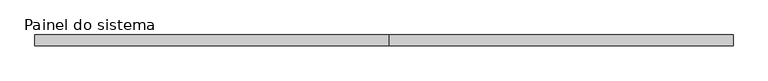
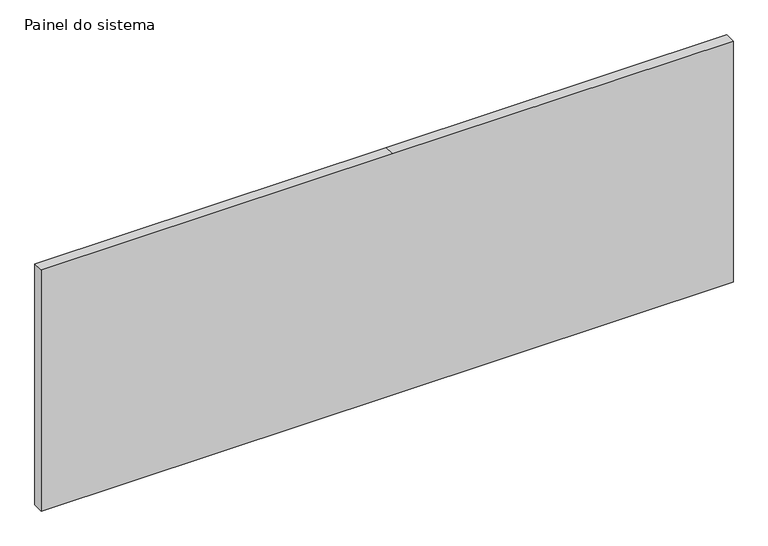
"""IFC4 building model written with IfcOpenShell, lengths in millimetres: plate geometry, Painel do sistema : Envidraçado."""

import ifcopenshell
import ifcopenshell.guid

model = None  # the IFC model being written
_history = None  # IfcOwnerHistory: only IFC2X3 demands one
_inside = {}  # id of a spatial element -> (the spatial element, [elements in it])
_under = {}  # id of a project, library or spatial element -> (it, [spatial elements below it])
_declared = {}  # id of a project -> (the project, [libraries it declares])
_typed = {}  # id of a type object -> (the type object, [elements of that type])
_made_of = {}  # id of a material, layer set ... -> (it, [elements and type objects made of it])


def new_model(schema):
    """Start an empty IFC model of exactly this schema.

    Asked for "IFC4X3", IfcOpenShell would pick the latest addendum, in which some entities
    have other attributes; the version numbers below select the first issue.
    IFC2X3 requires an IfcOwnerHistory on every rooted entity: one is made here for all.
    """
    global model, _history
    if schema == "IFC4X3":
        model = ifcopenshell.file(schema_version=(4, 3, 0, 0))
    else:
        model = ifcopenshell.file(schema=schema)
    _inside.clear()
    _under.clear()
    _declared.clear()
    _typed.clear()
    _made_of.clear()
    _history = None
    if model.schema == "IFC2X3":
        org = make("IfcOrganization", Name="unknown")
        user = make(
            "IfcPersonAndOrganization",
            ThePerson=make("IfcPerson", FamilyName="unknown"),
            TheOrganization=org,
        )
        app = make(
            "IfcApplication",
            ApplicationDeveloper=org,
            Version="unknown",
            ApplicationFullName="unknown",
            ApplicationIdentifier="unknown",
        )
        _history = make(
            "IfcOwnerHistory",
            OwningUser=user,
            OwningApplication=app,
            ChangeAction="ADDED",
            CreationDate=0,
        )
    return model


def make(cls, **values):
    """One entity of the class cls with the attributes given. An attribute that is None is left unset."""
    return model.create_entity(
        cls, **{name: value for name, value in values.items() if value is not None}
    )


def rooted(cls, **values):
    """An entity with a GlobalId (a new one), such as an element, a storey or a relation."""
    return make(cls, GlobalId=ifcopenshell.guid.new(), OwnerHistory=_history, **values)


def si_unit(unit_type, name, prefix=None):
    """IfcSIUnit, for example si_unit("LENGTHUNIT", "METRE", prefix="MILLI")."""
    return make("IfcSIUnit", UnitType=unit_type, Prefix=prefix, Name=name)


def assignment(units):
    """IfcUnitAssignment: the units of a project."""
    return None if units is None else make("IfcUnitAssignment", Units=units)


def point(xyz):
    """IfcCartesianPoint."""
    return None if xyz is None else make("IfcCartesianPoint", Coordinates=xyz)


def direction(xyz):
    """IfcDirection."""
    return None if xyz is None else make("IfcDirection", DirectionRatios=xyz)


def frame(location, z_axis=None, x_axis=None):
    """IfcAxis2Placement3D, a coordinate frame: its origin and axes. An axis left out is left unset."""
    return make(
        "IfcAxis2Placement3D",
        Location=point(location),
        Axis=direction(z_axis),
        RefDirection=direction(x_axis),
    )


def origin():
    """The frame at (0, 0, 0) with its axes left unset."""
    return frame((0.0, 0.0, 0.0))


def place(relative_to, where):
    """IfcLocalPlacement: puts the frame where relative to a parent placement (None: the world)."""
    return make(
        "IfcLocalPlacement", PlacementRelTo=relative_to, RelativePlacement=where
    )


def context(
    kind, dimensions, precision=None, world=None, true_north=None, identifier=None
):
    """IfcGeometricRepresentationContext, for example the 3D "Model" context."""
    return make(
        "IfcGeometricRepresentationContext",
        ContextIdentifier=identifier,
        ContextType=kind,
        CoordinateSpaceDimension=dimensions,
        Precision=precision,
        WorldCoordinateSystem=world,
        TrueNorth=true_north,
    )


def project(units=None, contexts=None):
    """IfcProject with its units and contexts."""
    return rooted(
        "IfcProject",
        Name="project",
        RepresentationContexts=contexts,
        UnitsInContext=assignment(units),
    )


def spatial(cls, under=None, at=None, **own):
    """A site, building, storey or space (cls), placed at a placement, below another one or the project."""
    s = rooted(cls, ObjectPlacement=at, **own)
    if under is not None:
        _under.setdefault(under.id(), (under, []))[1].append(s)
    return s


def polyline(points):
    """IfcPolyline through the points."""
    return make("IfcPolyline", Points=[point(p) for p in points])


def outline(outer, holes=None, kind="AREA"):
    """IfcArbitraryClosedProfileDef: a profile drawn as a closed curve; with holes, ...WithVoids."""
    if holes is None:
        return make("IfcArbitraryClosedProfileDef", ProfileType=kind, OuterCurve=outer)
    return make(
        "IfcArbitraryProfileDefWithVoids",
        ProfileType=kind,
        OuterCurve=outer,
        InnerCurves=holes,
    )


def extrude(swept, where, along, depth):
    """IfcExtrudedAreaSolid: the profile swept, set in the frame where, extruded along a direction by depth."""
    return make(
        "IfcExtrudedAreaSolid",
        SweptArea=swept,
        Position=where,
        ExtrudedDirection=direction(along),
        Depth=depth,
    )


def shape(context_of_items, identifier, shape_type, items):
    """IfcShapeRepresentation: the items that make up one representation, for example the "Body"."""
    return make(
        "IfcShapeRepresentation",
        ContextOfItems=context_of_items,
        RepresentationIdentifier=identifier,
        RepresentationType=shape_type,
        Items=items,
    )


def source(mapping_origin, context_of_items, identifier, shape_type, items):
    """IfcRepresentationMap: a shape defined once, which mapped items show again and again."""
    return make(
        "IfcRepresentationMap",
        MappingOrigin=mapping_origin,
        MappedRepresentation=shape(context_of_items, identifier, shape_type, items),
    )


def transform(
    local_origin,
    x_axis=None,
    y_axis=None,
    z_axis=None,
    scale=None,
    scale2=None,
    scale3=None,
    uniform=True,
):
    """IfcCartesianTransformationOperator3D, or its non-uniform kind. x_axis, y_axis, z_axis: its Axis1, 2, 3."""
    if uniform:
        return make(
            "IfcCartesianTransformationOperator3D",
            Axis1=direction(x_axis),
            Axis2=direction(y_axis),
            LocalOrigin=point(local_origin),
            Scale=scale,
            Axis3=direction(z_axis),
        )
    return make(
        "IfcCartesianTransformationOperator3DnonUniform",
        Axis1=direction(x_axis),
        Axis2=direction(y_axis),
        LocalOrigin=point(local_origin),
        Scale=scale,
        Axis3=direction(z_axis),
        Scale2=scale2,
        Scale3=scale3,
    )


def mapped(mapping_source, mapping_target):
    """IfcMappedItem: shows the shape of a source again, moved by a transform."""
    return make(
        "IfcMappedItem", MappingSource=mapping_source, MappingTarget=mapping_target
    )


def made_of(thing, what):
    """Note that an element or type object is made of a material, layer set ...; save() writes the relation."""
    if what is not None:
        _made_of.setdefault(what.id(), (what, []))[1].append(thing)
    return thing


def element(
    cls,
    number,
    at=None,
    inside=None,
    cuts=None,
    type_object=None,
    material=None,
    context=None,
    identifier="Body",
    shape_type=None,
    held_by="IfcProductDefinitionShape",
    body=None,
    shapes=None,
    **own,
):
    """One element of the class cls, such as IfcWall. Its Tag is "e" and its number.

    at: its placement. inside: the storey or other place that contains it. cuts: it is an
    opening in that element (IfcRelVoidsElement). A single representation is given by context,
    identifier, shape_type and body (its items); several are given by shapes. held_by: the class
    of the entity that holds the representations. save() writes the other relations.
    """
    e = rooted(cls, Tag="e%d" % number, ObjectPlacement=at, **own)
    if body is not None:
        shapes = [shape(context, identifier, shape_type, body)]
    if shapes is not None:
        e.Representation = make(held_by, Representations=shapes)
    if inside is not None:
        _inside.setdefault(inside.id(), (inside, []))[1].append(e)
    if cuts is not None:
        rooted(
            "IfcRelVoidsElement", RelatingBuildingElement=cuts, RelatedOpeningElement=e
        )
    if type_object is not None:
        _typed.setdefault(type_object.id(), (type_object, []))[1].append(e)
    return made_of(e, material)


def aggregate(whole, parts):
    """IfcRelAggregates: a whole, such as a stair, and the parts it consists of."""
    return rooted("IfcRelAggregates", RelatingObject=whole, RelatedObjects=parts)


def save(model, path):
    """Write the relations noted so far, then the file.

    IfcRelAggregates (storeys below a building ...), IfcRelContainedInSpatialStructure (elements
    in a storey), IfcRelDefinesByType, IfcRelAssociatesMaterial and IfcRelDeclares: one each for
    every whole, place, type object, material and project.
    """
    for whole, parts in _under.values():
        aggregate(whole, parts)
    for where, things in _inside.values():
        rooted(
            "IfcRelContainedInSpatialStructure",
            RelatedElements=things,
            RelatingStructure=where,
        )
    for kind, things in _typed.values():
        rooted("IfcRelDefinesByType", RelatedObjects=things, RelatingType=kind)
    for what, things in _made_of.values():
        rooted("IfcRelAssociatesMaterial", RelatedObjects=things, RelatingMaterial=what)
    for by, libraries in _declared.values():
        rooted("IfcRelDeclares", RelatingContext=by, RelatedDefinitions=libraries)
    model.write(path)


def painel_do_sistema_b00e55f7(model_context):
    return source(origin(), model_context, "Body", "SweptSolid", [
        extrude(outline(polyline([(0.0, -800.0500001), (0.0, 12.4999998), (0.0, 800.0500001), (590.0, 800.0500001), (590.0, 12.4999998), (590.0, -800.0500001), (0.0, -800.0500001)])), frame((0.0, -49.5, 0.0), z_axis=(0.0, 1.0, 0.0), x_axis=(0.0, 0.0, 1.0)), (0.0, 0.0, 1.0), 25.0),
    ])


if __name__ == "__main__":
    model = new_model("IFC4")
    model_context = context("Model", 3, world=origin())
    ifc_project = project(units=[si_unit("LENGTHUNIT", "METRE", prefix="MILLI")], contexts=[model_context])
    site = spatial("IfcSite", under=ifc_project)
    building = spatial("IfcBuilding", under=site)
    placement = place(None, origin())
    painel_do_sistema_shape = painel_do_sistema_b00e55f7(model_context)
    element("IfcPlate", 1, ObjectType="Painel do sistema : Envidraçado", at=placement, inside=building, context=model_context, shape_type="MappedRepresentation", body=[
        mapped(painel_do_sistema_shape, transform((0.0, 0.0, 0.0), x_axis=(1.0, 0.0, 0.0), y_axis=(0.0, 1.0, 0.0), z_axis=(0.0, 0.0, 1.0))),
    ])
    save(model, "model.ifc")

# Revit data of these elements
# Type "Painel do sistema : Envidraçado"
#   Construction Type Id = "GSP4R"
#   Analytic Construction = "Vidraça única Pilkington 1/8 pol"
#   Visual Light Transmittance = 0.9
#   Solar Heat Gain Coefficient = 0.86
#   Heat Transfer Coefficient (U) = 6.7069 W/(m²·K)
# Element 1 (IfcPlate, "Painel do sistema : Envidraçado")
#   Materials on its faces: ".VIDRO GENÉRICO"
# Materials
#   ".VIDRO GENÉRICO": class ".CC_VIDRO", colour RGB 0 128 192, transparency 0.9, Description = "Vidro comum", Cost = 0
